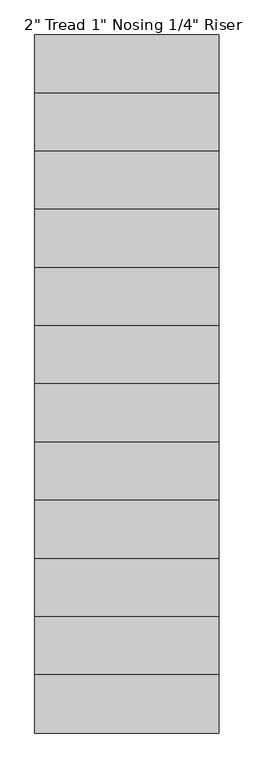
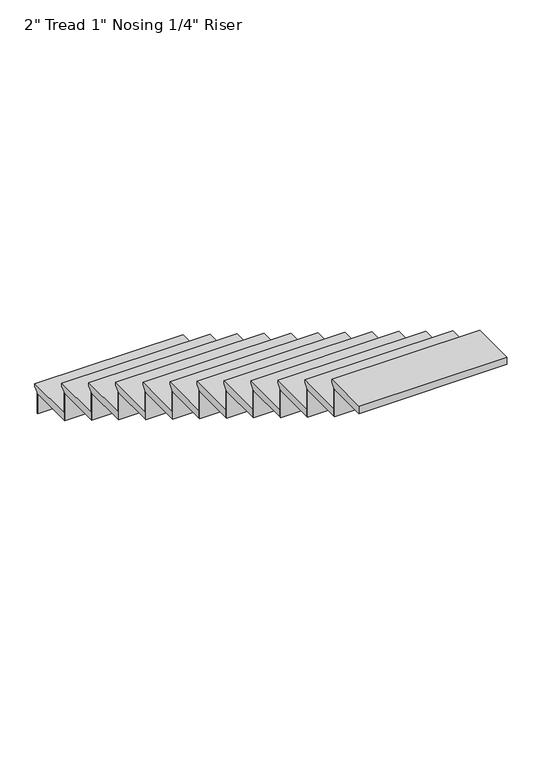
"""IFC4 building model written with IfcOpenShell, lengths in millimetres: stair flight geometry."""

from ifc_helpers import new_model, si_unit, frame, origin, place, context, project, spatial, polyline, outline, extrude, source, transform, mapped, element, save


def stair_flight_88c5a219(model_context):
    return source(origin(), model_context, "Body", "SweptSolid", [
        extrude(outline(polyline([(-3156.3830088, -2250.8307692), (-2826.1830088, -2250.8307692), (-2826.1830088, -2269.8807692), (-2851.5830088, -2295.2807692), (-2851.5830088, -2301.6307692), (-3156.3830088, -2301.6307692), (-3156.3830088, -2250.8307692)])), frame((31460.7652986, 0.0, 0.0), z_axis=(1.0, 0.0, 0.0), x_axis=(0.0, 1.0, 0.0)), (0.0, 0.0, 1.0), 965.2),
        extrude(outline(polyline([(31460.7652986, -2857.9330088), (31460.7652986, -2851.5830088), (32425.9652986, -2851.5830088), (32425.9652986, -2857.9330088), (31460.7652986, -2857.9330088)])), frame((0.0, 0.0, -2438.4), z_axis=(0.0, 0.0, 1.0), x_axis=(1.0, 0.0, 0.0)), (0.0, 0.0, 1.0), 136.7692308),
        extrude(outline(polyline([(31460.7652986, -3162.7330088), (31460.7652986, -3156.3830088), (32425.9652986, -3156.3830088), (32425.9652986, -3162.7330088), (31460.7652986, -3162.7330088)])), frame((0.0, 0.0, -2301.6307692), z_axis=(0.0, 0.0, 1.0), x_axis=(1.0, 0.0, 0.0)), (0.0, 0.0, 1.0), 187.5692308),
        extrude(outline(polyline([(-3461.1830088, -2063.2615385), (-3130.9830088, -2063.2615385), (-3130.9830088, -2082.3115385), (-3156.3830088, -2107.7115385), (-3156.3830088, -2114.0615385), (-3461.1830088, -2114.0615385), (-3461.1830088, -2063.2615385)])), frame((31460.7652986, 0.0, 0.0), z_axis=(1.0, 0.0, 0.0), x_axis=(0.0, 1.0, 0.0)), (0.0, 0.0, 1.0), 965.2),
        extrude(outline(polyline([(31460.7652986, -3467.5330088), (31460.7652986, -3461.1830088), (32425.9652986, -3461.1830088), (32425.9652986, -3467.5330088), (31460.7652986, -3467.5330088)])), frame((0.0, 0.0, -2114.0615385), z_axis=(0.0, 0.0, 1.0), x_axis=(1.0, 0.0, 0.0)), (0.0, 0.0, 1.0), 187.5692308),
        extrude(outline(polyline([(-3765.9830088, -1875.6923077), (-3435.7830088, -1875.6923077), (-3435.7830088, -1894.7423077), (-3461.1830088, -1920.1423077), (-3461.1830088, -1926.4923077), (-3765.9830088, -1926.4923077), (-3765.9830088, -1875.6923077)])), frame((31460.7652986, 0.0, 0.0), z_axis=(1.0, 0.0, 0.0), x_axis=(0.0, 1.0, 0.0)), (0.0, 0.0, 1.0), 965.2),
        extrude(outline(polyline([(31460.7652986, -3772.3330088), (31460.7652986, -3765.9830088), (32425.9652986, -3765.9830088), (32425.9652986, -3772.3330088), (31460.7652986, -3772.3330088)])), frame((0.0, 0.0, -1926.4923077), z_axis=(0.0, 0.0, 1.0), x_axis=(1.0, 0.0, 0.0)), (0.0, 0.0, 1.0), 187.5692308),
        extrude(outline(polyline([(-4070.7830088, -1688.1230769), (-3740.5830088, -1688.1230769), (-3740.5830088, -1707.1730769), (-3765.9830088, -1732.5730769), (-3765.9830088, -1738.9230769), (-4070.7830088, -1738.9230769), (-4070.7830088, -1688.1230769)])), frame((31460.7652986, 0.0, 0.0), z_axis=(1.0, 0.0, 0.0), x_axis=(0.0, 1.0, 0.0)), (0.0, 0.0, 1.0), 965.2),
        extrude(outline(polyline([(31460.7652986, -4077.1330088), (31460.7652986, -4070.7830088), (32425.9652986, -4070.7830088), (32425.9652986, -4077.1330088), (31460.7652986, -4077.1330088)])), frame((0.0, 0.0, -1738.9230769), z_axis=(0.0, 0.0, 1.0), x_axis=(1.0, 0.0, 0.0)), (0.0, 0.0, 1.0), 187.5692308),
        extrude(outline(polyline([(-4375.5830088, -1500.5538462), (-4045.3830088, -1500.5538462), (-4045.3830088, -1519.6038462), (-4070.7830088, -1545.0038462), (-4070.7830088, -1551.3538462), (-4375.5830088, -1551.3538462), (-4375.5830088, -1500.5538462)])), frame((31460.7652986, 0.0, 0.0), z_axis=(1.0, 0.0, 0.0), x_axis=(0.0, 1.0, 0.0)), (0.0, 0.0, 1.0), 965.2),
        extrude(outline(polyline([(31460.7652986, -4381.9330088), (31460.7652986, -4375.5830088), (32425.9652986, -4375.5830088), (32425.9652986, -4381.9330088), (31460.7652986, -4381.9330088)])), frame((0.0, 0.0, -1551.3538462), z_axis=(0.0, 0.0, 1.0), x_axis=(1.0, 0.0, 0.0)), (0.0, 0.0, 1.0), 187.5692308),
        extrude(outline(polyline([(-4680.3830088, -1312.9846154), (-4350.1830088, -1312.9846154), (-4350.1830088, -1332.0346154), (-4375.5830088, -1357.4346154), (-4375.5830088, -1363.7846154), (-4680.3830088, -1363.7846154), (-4680.3830088, -1312.9846154)])), frame((31460.7652986, 0.0, 0.0), z_axis=(1.0, 0.0, 0.0), x_axis=(0.0, 1.0, 0.0)), (0.0, 0.0, 1.0), 965.2),
        extrude(outline(polyline([(31460.7652986, -4686.7330088), (31460.7652986, -4680.3830088), (32425.9652986, -4680.3830088), (32425.9652986, -4686.7330088), (31460.7652986, -4686.7330088)])), frame((0.0, 0.0, -1363.7846154), z_axis=(0.0, 0.0, 1.0), x_axis=(1.0, 0.0, 0.0)), (0.0, 0.0, 1.0), 187.5692308),
        extrude(outline(polyline([(-4985.1830088, -1125.4153846), (-4654.9830088, -1125.4153846), (-4654.9830088, -1144.4653846), (-4680.3830088, -1169.8653846), (-4680.3830088, -1176.2153846), (-4985.1830088, -1176.2153846), (-4985.1830088, -1125.4153846)])), frame((31460.7652986, 0.0, 0.0), z_axis=(1.0, 0.0, 0.0), x_axis=(0.0, 1.0, 0.0)), (0.0, 0.0, 1.0), 965.2),
        extrude(outline(polyline([(31460.7652986, -4991.5330088), (31460.7652986, -4985.1830088), (32425.9652986, -4985.1830088), (32425.9652986, -4991.5330088), (31460.7652986, -4991.5330088)])), frame((0.0, 0.0, -1176.2153846), z_axis=(0.0, 0.0, 1.0), x_axis=(1.0, 0.0, 0.0)), (0.0, 0.0, 1.0), 187.5692308),
        extrude(outline(polyline([(-5289.9830088, -937.8461538), (-4959.7830088, -937.8461538), (-4959.7830088, -956.8961538), (-4985.1830088, -982.2961538), (-4985.1830088, -988.6461538), (-5289.9830088, -988.6461538), (-5289.9830088, -937.8461538)])), frame((31460.7652986, 0.0, 0.0), z_axis=(1.0, 0.0, 0.0), x_axis=(0.0, 1.0, 0.0)), (0.0, 0.0, 1.0), 965.2),
        extrude(outline(polyline([(31460.7652986, -5296.3330088), (31460.7652986, -5289.9830088), (32425.9652986, -5289.9830088), (32425.9652986, -5296.3330088), (31460.7652986, -5296.3330088)])), frame((0.0, 0.0, -988.6461538), z_axis=(0.0, 0.0, 1.0), x_axis=(1.0, 0.0, 0.0)), (0.0, 0.0, 1.0), 187.5692308),
        extrude(outline(polyline([(-5594.7830088, -750.2769231), (-5264.5830088, -750.2769231), (-5264.5830088, -769.3269231), (-5289.9830088, -794.7269231), (-5289.9830088, -801.0769231), (-5594.7830088, -801.0769231), (-5594.7830088, -750.2769231)])), frame((31460.7652986, 0.0, 0.0), z_axis=(1.0, 0.0, 0.0), x_axis=(0.0, 1.0, 0.0)), (0.0, 0.0, 1.0), 965.2),
        extrude(outline(polyline([(31460.7652986, -5601.1330088), (31460.7652986, -5594.7830088), (32425.9652986, -5594.7830088), (32425.9652986, -5601.1330088), (31460.7652986, -5601.1330088)])), frame((0.0, 0.0, -801.0769231), z_axis=(0.0, 0.0, 1.0), x_axis=(1.0, 0.0, 0.0)), (0.0, 0.0, 1.0), 187.5692308),
        extrude(outline(polyline([(-5899.5830088, -562.7076923), (-5569.3830088, -562.7076923), (-5569.3830088, -581.7576923), (-5594.7830088, -607.1576923), (-5594.7830088, -613.5076923), (-5899.5830088, -613.5076923), (-5899.5830088, -562.7076923)])), frame((31460.7652986, 0.0, 0.0), z_axis=(1.0, 0.0, 0.0), x_axis=(0.0, 1.0, 0.0)), (0.0, 0.0, 1.0), 965.2),
        extrude(outline(polyline([(31460.7652986, -5905.9330088), (31460.7652986, -5899.5830088), (32425.9652986, -5899.5830088), (32425.9652986, -5905.9330088), (31460.7652986, -5905.9330088)])), frame((0.0, 0.0, -613.5076923), z_axis=(0.0, 0.0, 1.0), x_axis=(1.0, 0.0, 0.0)), (0.0, 0.0, 1.0), 187.5692308),
        extrude(outline(polyline([(-6204.3830088, -375.1384615), (-5874.1830088, -375.1384615), (-5874.1830088, -394.1884615), (-5899.5830088, -419.5884615), (-5899.5830088, -425.9384615), (-6204.3830088, -425.9384615), (-6204.3830088, -375.1384615)])), frame((31460.7652986, 0.0, 0.0), z_axis=(1.0, 0.0, 0.0), x_axis=(0.0, 1.0, 0.0)), (0.0, 0.0, 1.0), 965.2),
        extrude(outline(polyline([(31460.7652986, -6210.7330088), (31460.7652986, -6204.3830088), (32425.9652986, -6204.3830088), (32425.9652986, -6210.7330088), (31460.7652986, -6210.7330088)])), frame((0.0, 0.0, -425.9384615), z_axis=(0.0, 0.0, 1.0), x_axis=(1.0, 0.0, 0.0)), (0.0, 0.0, 1.0), 187.5692308),
        extrude(outline(polyline([(-6483.7830088, -187.5692308), (-6178.9830088, -187.5692308), (-6178.9830088, -206.6192308), (-6204.3830088, -232.0192308), (-6204.3830088, -238.3692308), (-6483.7830088, -238.3692308), (-6483.7830088, -187.5692308)])), frame((31460.7652986, 0.0, 0.0), z_axis=(1.0, 0.0, 0.0), x_axis=(0.0, 1.0, 0.0)), (0.0, 0.0, 1.0), 965.2),
    ])


if __name__ == "__main__":
    model = new_model("IFC4")
    model_context = context("Model", 3, world=origin())
    ifc_project = project(units=[si_unit("LENGTHUNIT", "METRE", prefix="MILLI")], contexts=[model_context])
    site = spatial("IfcSite", under=ifc_project)
    building = spatial("IfcBuilding", under=site)
    placement = place(None, origin())
    stair_flight_shape = stair_flight_88c5a219(model_context)
    element("IfcStairFlight", 1, ObjectType="2\" Tread 1\" Nosing 1/4\" Riser", at=placement, inside=building, context=model_context, shape_type="MappedRepresentation", body=[
        mapped(stair_flight_shape, transform((0.0, 0.0, 0.0), x_axis=(1.0, 0.0, 0.0), y_axis=(0.0, 1.0, 0.0), z_axis=(0.0, 0.0, 1.0))),
    ])
    save(model, "model.ifc")

# Revit data of these elements
# Element 1 (IfcStairFlight, "2\" Tread 1\" Nosing 1/4\" Riser")
#   Materials on its faces: "Default Floor"
# Materials
#   "Default Floor": class "Miscellaneous", colour RGB 255 255 255, transparency 0, Cost = 0
